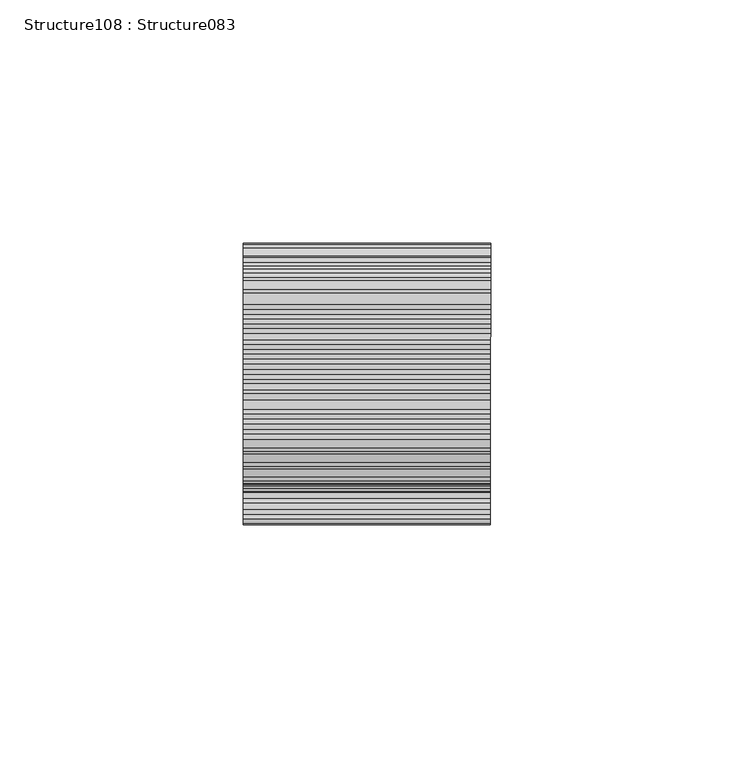
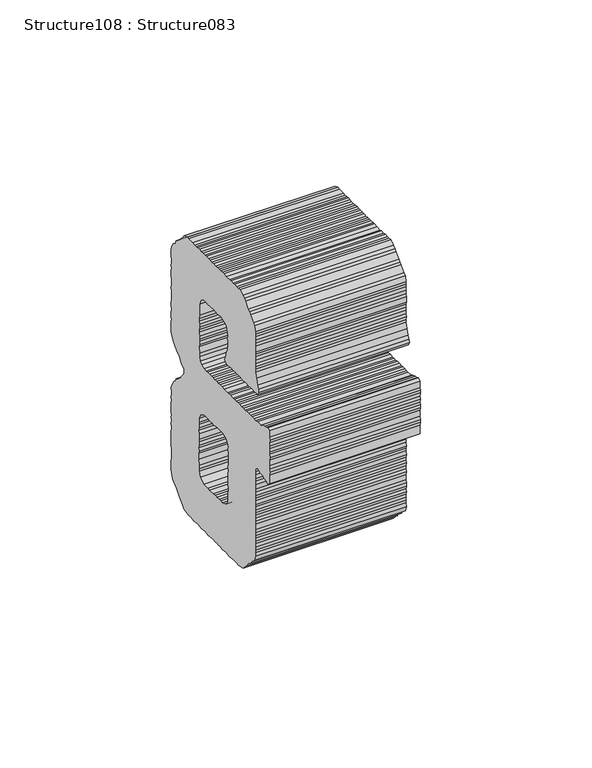
"""IFC4 building model written with IfcOpenShell, lengths in millimetres: proxy geometry, Structure108 : Structure083."""

from ifc_helpers import new_model, si_unit, frame, origin, place, context, project, spatial, polyline, outline, extrude, source, transform, mapped, element, save


def structure108_structure083_72f0dcc1(model_context):
    return source(origin(), model_context, "Body", "SweptSolid", [
        extrude(outline(polyline([(2.0811665, 0.0), (2.9845827, 0.2618803), (3.8993851, 0.1334309), (5.0653934, 0.1334309), (5.9801957, 0.0), (7.1465598, 0.1334309), (7.922594, 0.0), (9.0982094, 0.0), (10.2638618, 0.2618803), (11.3028439, 0.1334309), (12.3450283, 0.2618803), (13.3836546, 0.0), (15.072712, -0.7806599), (16.3682373, -2.3373539), (17.4104217, -2.7280396), (18.0572948, -3.7655984), (18.839022, -4.4131831), (19.362427, -5.0653934), (20.2676224, -5.8460532), (21.0529078, -6.7555183), (21.9570357, -7.4077287), (22.609246, -9.2263031), (22.4818639, -10.0023373), (22.4818639, -12.3446725), (22.3466539, -13.3825871), (22.3466539, -14.4205018), (22.609246, -15.3296111), (22.609246, -16.3675257), (22.3466539, -17.2816165), (22.3466539, -18.3195311), (22.4818639, -19.6143446), (22.609246, -20.5284353), (22.4818639, -21.56635), (22.4818639, -22.4804407), (22.3466539, -23.5183553), (22.4818639, -24.55627), (22.3466539, -25.7272597), (22.3466539, -26.7651743), (22.4818639, -27.8030889), (22.4818639, -28.5837487), (22.609246, -29.8835437), (22.609246, -30.6642035), (22.3466539, -31.9639986), (22.3466539, -33.9110225), (22.609246, -34.8204876), (22.3466539, -35.8633837), (22.609246, -36.9009425), (22.4818639, -38.0673065), (22.4818639, -38.9767717), (22.609246, -40.1477613), (21.6940878, -41.8378863), (21.0529078, -42.6139205), (20.2676224, -43.1327), (18.582123, -44.8228249), (18.0572948, -45.6038405), (17.4104217, -46.1226199), (15.5922031, -47.8127448), (14.9392811, -48.5934047), (13.1214183, -49.1125398), (12.2158672, -48.9840903), (11.3028439, -48.9840903), (10.1368356, -49.1125398), (8.9647784, -49.1125398), (7.922594, -49.2459707), (5.8474764, -49.2459707), (5.0653934, -49.1125398), (4.0267671, -48.9840903), (2.9845827, -49.1125398), (1.6911924, -48.9840903), (0.7817272, -49.2459707), (-0.3899741, -48.9840903), (-1.2990834, -49.1125398), (-3.246819, -49.6313193), (-5.3276296, -50.1500986), (-6.3644768, -50.8026648), (-7.5361781, -50.9261328), (-8.5790742, -50.4119791), (-8.5790742, -49.6313193), (-8.7078795, -48.4599737), (-8.4456433, -47.2939654), (-8.4456433, -46.2510694), (-8.7078795, -45.3465857), (-8.4456433, -44.175596), (-8.4456433, -43.2661309), (-8.7078795, -42.2282163), (-8.4456433, -40.1477613), (-8.4456433, -39.238652), (-8.5790742, -38.195756), (-8.4456433, -37.0293919), (-8.7078795, -35.8633837), (-8.4456433, -34.9489371), (-8.4456433, -34.0398278), (-8.7078795, -33.0019132), (-8.4456433, -31.9639986), (-7.663916, -31.0499079), (-6.6270688, -31.7021181), (-4.2836661, -32.0924481), (-3.5097668, -32.7400327), (-1.2990834, -33.0019132), (-0.3899741, -33.0019132), (1.0421844, -32.7400327), (1.8185744, -33.0019132), (2.9845827, -32.8684823), (4.8031571, -32.2208976), (5.4553675, -31.7021181), (5.8474764, -29.7501128), (6.1079336, -28.8456291), (5.9801957, -27.669658), (5.8474764, -26.5032939), (5.9801957, -25.7272597), (6.1079336, -24.422839), (5.9801957, -23.3849244), (6.1079336, -22.4804407), (5.8474764, -21.3044696), (6.1079336, -20.1381055), (6.1079336, -19.1001909), (5.0653934, -17.1481855), (2.9845827, -16.3675257), (-0.9091093, -16.3675257), (-2.2046346, -16.1106267), (-3.1176578, -16.1106267), (-4.1559283, -16.2390762), (-5.1988243, -16.2390762), (-6.2370947, -16.1106267), (-7.140511, -16.1106267), (-8.4456433, -16.3675257), (-9.3547526, -16.3675257), (-10.2642177, -16.2390762), (-11.435919, -16.2390762), (-12.3393353, -16.1106267), (-14.4205017, -16.3675257), (-15.7195851, -16.3675257), (-17.0243616, -16.7578556), (-17.6673207, -17.6673207), (-18.319531, -18.9717414), (-18.5824789, -20.1381055), (-18.319531, -21.1760201), (-18.4529619, -22.0851294), (-18.319531, -23.3849244), (-18.4529619, -24.16594), (-18.5824789, -25.2034988), (-18.319531, -26.5032939), (-18.4529619, -27.2839537), (-18.319531, -28.4552992), (-18.4529619, -29.4932138), (-18.5824789, -30.6642035), (-18.5824789, -32.7400327), (-18.4529619, -33.649142), (-18.4529619, -34.5586072), (-18.5824789, -35.8633837), (-18.319531, -36.9009425), (-18.4529619, -37.8054262), (-18.4529619, -38.8479664), (-18.319531, -39.885881), (-18.5824789, -41.052245), (-18.4529619, -41.9663358), (-18.5824789, -42.8758009), (-18.319531, -43.9137156), (-18.319531, -45.0847053), (-18.4529619, -46.2510694), (-18.319531, -47.1651601), (-18.319531, -48.3315242), (-18.5824789, -49.2459707), (-18.319531, -50.2835295), (-18.319531, -52.2309093), (-17.6673207, -53.1400187), (-17.2773466, -54.4348322), (-17.1478297, -55.4777282), (-16.6286944, -56.3868375), (-17.2773466, -57.2963027), (-19.6186144, -57.2963027), (-20.4003417, -57.5532016), (-21.4371888, -57.4297336), (-22.736628, -57.2963027), (-23.6478722, -57.4297336), (-24.8174387, -57.2963027), (-25.5934729, -57.4297336), (-26.6360131, -57.5532016), (-27.6746394, -57.2963027), (-29.75545, -57.2963027), (-30.9214583, -57.4297336), (-31.8344816, -57.5532016), (-33.1300068, -57.2963027), (-36.1202826, -57.2963027), (-36.7724929, -56.3868375), (-36.2494437, -55.3489229), (-36.1202826, -54.3063827), (-35.5968776, -53.1400187), (-35.4677165, -52.1021039), (-34.8208434, -50.2835295), (-35.8576906, -49.1125398), (-36.899875, -49.1125398), (-37.9385012, -48.9840903), (-39.2379404, -49.1125398), (-40.1470497, -49.1125398), (-41.3187511, -49.2459707), (-43.1373255, -48.9840903), (-44.1759518, -48.9840903), (-45.3455182, -49.2459707), (-46.2567624, -48.9840903), (-47.1601787, -49.1125398), (-48.4653109, -49.2459707), (-49.3687272, -49.1125398), (-50.5404285, -48.9840903), (-51.3221558, -49.2459707), (-52.3590029, -49.1125398), (-53.5307043, -48.9840903), (-54.4398136, -49.2459707), (-55.6058219, -49.1125398), (-57.4243963, -49.1125398), (-58.4665807, -49.2459707), (-59.6386379, -49.2459707), (-60.6769083, -48.9840903), (-61.5863734, -49.2459707), (-62.6228648, -48.9840903), (-63.665405, -49.1125398), (-64.8331924, -48.9840903), (-65.7426575, -48.9840903), (-66.912224, -49.2459707), (-68.7268844, -48.5934047), (-69.2502894, -47.8127448), (-70.1593987, -46.9032797), (-71.068508, -46.3845003), (-71.7210742, -45.3465857), (-72.2345163, -44.6943753), (-73.2788356, -44.175596), (-74.0587838, -43.1327), (-75.6147662, -41.8378863), (-76.0065194, -40.0143304), (-76.1339014, -39.1102026), (-76.0065194, -37.9388571), (-76.0065194, -36.1153012), (-76.2673323, -34.9489371), (-76.2673323, -33.9110225), (-76.0065194, -32.8684823), (-76.0065194, -31.9639986), (-76.2673323, -30.9264397), (-76.2673323, -29.6216633), (-76.0065194, -28.7121982), (-76.1339014, -27.669658), (-76.0065194, -26.5032939), (-76.1339014, -25.7272597), (-76.0065194, -24.55627), (-76.0065194, -22.609246), (-76.2673323, -21.6947994), (-76.1339014, -20.3999859), (-76.0065194, -19.4858951), (-76.0065194, -18.4479805), (-76.2673323, -17.5434968), (-76.0065194, -15.463042), (-76.0065194, -14.1632469), (-76.2673323, -13.2491562), (-76.0065194, -12.0827921), (-76.0065194, -11.3021323), (-76.1339014, -10.0023373), (-76.0065194, -8.9644227), (-75.4873841, -7.4077287), (-74.8405111, -6.6270688), (-73.9257087, -5.7176037), (-72.4971084, -4.2893592), (-71.8502353, -3.7655984), (-70.8080509, -2.8564891), (-69.2502894, -1.2948136), (-68.7268844, -0.6522104), (-66.912224, 0.0), (-65.8700396, 0.1334309), (-64.7040313, 0.1334309), (-63.9240831, 0.2618803), (-62.7523817, 0.2618803), (-61.8468306, 0.0), (-58.4665807, 0.0), (-57.4243963, 0.2618803), (-55.4766608, 0.2618803), (-54.5671956, 0.1334309), (-53.6637794, 0.1334309), (-52.3590029, 0.2618803), (-51.3221558, 0.0), (-50.5404285, 0.0), (-49.3687272, 0.1334309), (-48.4653109, 0.0), (-47.1601787, 0.1334309), (-46.3841445, 0.0), (-45.3455182, 0.2618803), (-44.4324949, 0.2618803), (-43.1373255, 0.1334309), (-42.0947853, 0.2618803), (-41.185676, 0.0), (-40.0196677, 0.2618803), (-38.9771275, 0.0), (-37.9385012, 0.0), (-37.0293919, 0.2618803), (-35.8576906, 0.0), (-34.4290902, -0.7806599), (-33.5199809, -1.4282446), (-32.7400327, -2.2089043), (-31.8344816, -2.7280396), (-31.3114324, -3.7655984), (-30.4080162, -4.2893592), (-29.6223749, -5.3272738), (-28.8406477, -5.9794841), (-27.9372314, -6.7555183), (-27.1515902, -7.2742978), (-25.7229898, -7.2742978), (-24.5569815, -5.8460532), (-23.7752543, -5.3272738), (-22.866145, -4.546614), (-21.4371888, -2.9849386), (-20.5241656, -2.0804549), (-19.2286403, -0.7806599), (-17.5378038, 0.0), (-16.3717955, 0.1334309), (-13.2541376, 0.1334309), (-12.2119532, 0.0), (-11.435919, 0.1334309), (-10.1347007, 0.1334309), (-8.4456433, 0.0), (-7.4034588, 0.1334309), (-6.2370947, 0.1334309), (-5.3276296, 0.0), (-2.2046346, 0.0), (-1.0386263, 0.2618803), (0.0, 0.0), (2.0811665, 0.0)]), holes=[polyline([(-35.4677165, -31.7021181), (-34.8208434, -29.8835437), (-34.8208434, -28.7121982), (-34.9482254, -27.9315384), (-34.8208434, -26.6317434), (-34.9482254, -25.4653793), (-35.0816564, -24.55627), (-34.8208434, -23.5183553), (-35.0816564, -22.4804407), (-34.8208434, -21.1760201), (-34.9482254, -20.3999859), (-34.8208434, -19.1001909), (-35.7303085, -17.2816165), (-37.6759092, -16.3675257), (-38.9771275, -16.3675257), (-39.8865926, -16.2390762), (-40.9230839, -16.3675257), (-42.0947853, -16.1106267), (-43.1373255, -16.3675257), (-45.0850611, -16.3675257), (-46.1215524, -16.2390762), (-47.2936096, -16.3675257), (-48.2027189, -16.1106267), (-49.3687272, -16.3675257), (-50.1543684, -16.1106267), (-52.3590029, -16.1106267), (-54.4398136, -16.3675257), (-55.6058219, -16.3675257), (-56.6483621, -16.2390762), (-58.2061236, -17.019736), (-59.505207, -19.1001909), (-59.505207, -21.4379005), (-59.6386379, -22.2185603), (-59.6386379, -24.422839), (-59.3760458, -25.7272597), (-59.505207, -26.6317434), (-59.505207, -27.9315384), (-59.3760458, -28.8456291), (-59.505207, -29.8835437), (-58.8529967, -31.7021181), (-58.3391987, -32.3543285), (-56.5209801, -32.7400327), (-55.4766608, -32.8684823), (-54.3067385, -32.8684823), (-53.2681123, -33.0019132), (-52.2316209, -33.0019132), (-51.4495378, -32.8684823), (-50.4073534, -32.7400327), (-49.2413451, -32.8684823), (-47.2936096, -32.8684823), (-45.9941704, -33.0019132), (-45.2181362, -32.7400327), (-43.9133597, -33.0019132), (-40.0196677, -33.0019132), (-38.8479663, -32.7400327), (-37.6759092, -33.0019132), (-36.2494437, -32.2208976), (-35.4677165, -31.7021181)])]), frame((-56111.6870498, 290909.9870532, -299.204062), z_axis=(-0.9999998917542984, 0.00046528635450596156, 0.0), x_axis=(0.0, 0.0, 1.0)), (0.0, 0.0, 1.0), 50.8),
    ])


if __name__ == "__main__":
    model = new_model("IFC4")
    model_context = context("Model", 3, world=origin())
    ifc_project = project(units=[si_unit("LENGTHUNIT", "METRE", prefix="MILLI")], contexts=[model_context])
    site = spatial("IfcSite", under=ifc_project)
    building = spatial("IfcBuilding", under=site)
    placement = place(None, origin())
    structure108_structure083_shape = structure108_structure083_72f0dcc1(model_context)
    element("IfcBuildingElementProxy", 1, Name="Structure108 : Structure083", ObjectType="Structure108 : Structure083", at=placement, inside=building, context=model_context, shape_type="MappedRepresentation", body=[
        mapped(structure108_structure083_shape, transform((0.0, 0.0, 0.0), x_axis=(1.0, 0.0, 0.0), y_axis=(0.0, 1.0, 0.0), z_axis=(0.0, 0.0, 1.0))),
    ])
    save(model, "model.ifc")

# Revit data of these elements
# Type "Structure108 : Structure083"
#   NameOverride = "Structure083"
# Element 1 (IfcBuildingElementProxy, "Structure108 : Structure083")
#   Materials on its faces: "BRUSHED ALUMINUM LETTERING"
# Materials
#   "BRUSHED ALUMINUM LETTERING": class "Unassigned", colour RGB 169 181 186, transparency 0, Cost = 0
